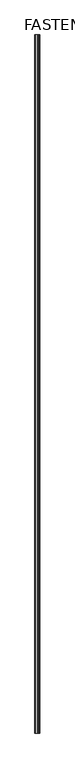
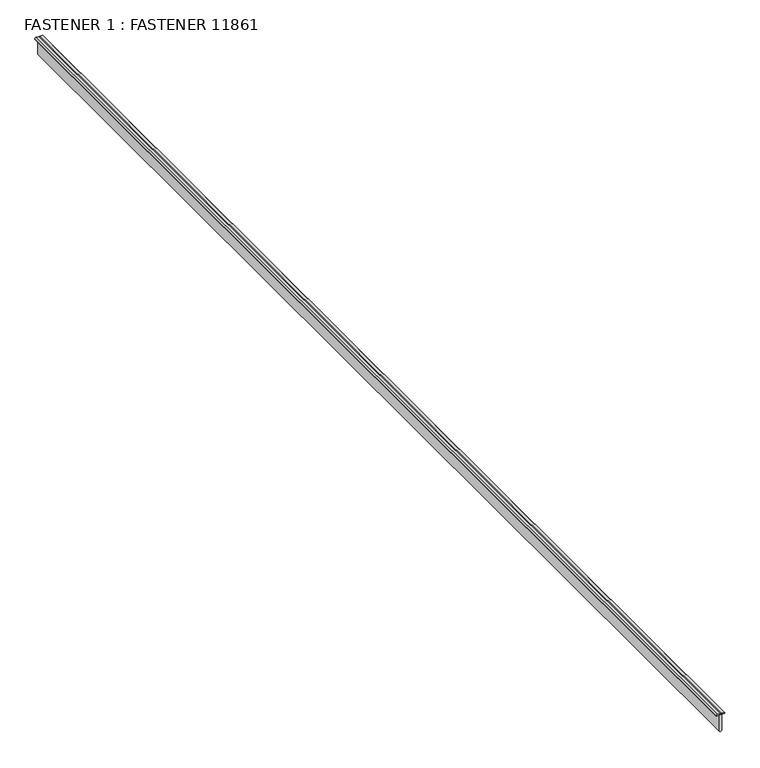
"""IFC4 building model written with IfcOpenShell, lengths in millimetres: proxy geometry, FASTENER 1 : FASTENER 11861."""

from ifc_helpers import new_model, si_unit, frame, origin, place, context, project, spatial, polyline, outline, extrude, source, transform, mapped, element, save


def fastener_1_fastener_11861_40db04d7(model_context):
    return source(origin(), model_context, "Body", "SweptSolid", [
        extrude(outline(polyline([(42551.3049701, 5981.517626), (42579.6987049, 5981.517626), (42579.6987049, 5977.3107075), (42550.7399648, 5977.3107075), (42549.1244121, 5978.9677221), (42551.3049701, 5981.517626)])), frame((0.0, -1052.8906574, 0.0), z_axis=(0.0, 1.0, 0.0), x_axis=(0.0, 0.0, 1.0)), (0.0, 0.0, 1.0), 1999.85),
        extrude(outline(polyline([(42580.5349921, 5972.2779845), (42579.6987049, 5972.2671879), (42579.6987049, 5986.5634932), (42580.508527, 5986.5634932), (42582.1023984, 5985.3247911), (42582.1023984, 5980.4457092), (42580.1167322, 5980.0391089), (42580.1167322, 5978.792004), (42581.7222633, 5978.792004), (42582.1288635, 5973.5166866), (42580.5349921, 5972.2779845)])), frame((0.0, -1052.8906574, 0.0), z_axis=(0.0, 1.0, 0.0), x_axis=(0.0, 0.0, 1.0)), (0.0, 0.0, 1.0), 1999.85),
    ])


if __name__ == "__main__":
    model = new_model("IFC4")
    model_context = context("Model", 3, world=origin())
    ifc_project = project(units=[si_unit("LENGTHUNIT", "METRE", prefix="MILLI")], contexts=[model_context])
    site = spatial("IfcSite", under=ifc_project)
    building = spatial("IfcBuilding", under=site)
    placement = place(None, origin())
    fastener_1_fastener_11861_shape = fastener_1_fastener_11861_40db04d7(model_context)
    element("IfcBuildingElementProxy", 1, Name="FASTENER 1 : FASTENER 11861", ObjectType="FASTENER 1 : FASTENER 11861", at=placement, inside=building, context=model_context, shape_type="MappedRepresentation", body=[
        mapped(fastener_1_fastener_11861_shape, transform((0.0, 0.0, 0.0), x_axis=(1.0, 0.0, 0.0), y_axis=(0.0, 1.0, 0.0), z_axis=(0.0, 0.0, 1.0))),
    ])
    save(model, "model.ifc")

# Revit data of these elements
# Type "FASTENER 1 : FASTENER 11861"
#   NameOverride = "FASTENER"
# Element 1 (IfcBuildingElementProxy, "FASTENER 1 : FASTENER 11861")
#   Materials on its faces: "ENGINEERED PANCAKE HEAD FASTENER (NOT BY AEP-SPAN) @ 12\" O.C."
# Materials
#   "ENGINEERED PANCAKE HEAD FASTENER (NOT BY AEP-SPAN) @ 12\" O.C.": class "Unassigned", colour RGB 255 255 255, transparency 0
